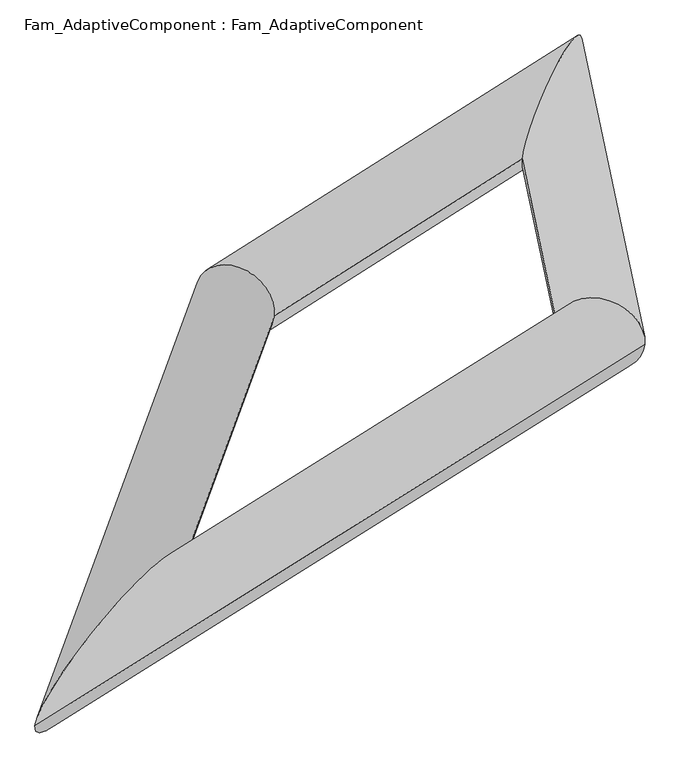
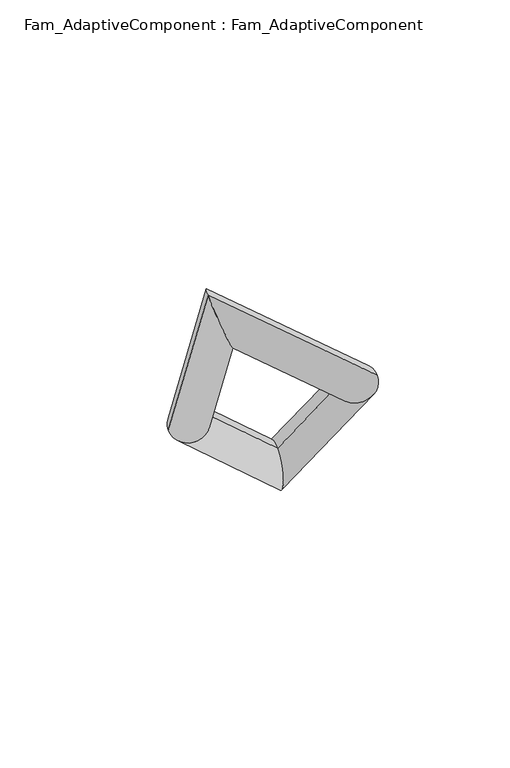
"""IFC4 building model written with IfcOpenShell, lengths in millimetres: proxy geometry, Fam_AdaptiveComponent : Fam_AdaptiveComponent."""

from ifc_helpers import new_model, si_unit, frame, origin, place, context, project, spatial, ellipse_curve, source, transform, mapped, element, save
from ifc_brep_helpers import cylinder_surface, advanced_brep


def fam_adaptivecomponent_fam_adaptivecomponent_cf6aee74(model_context):
    return source(origin(), model_context, "Body", "AdvancedBrep", [
        advanced_brep(
        [(4475.999331, 1861.8658467, -16792.1550666), (3077.0233369, 8482.3914405, -26020.1836237), (5467.6276173, 13102.4870202, -32934.2739452), (8018.1342606, 1032.4482346, -16110.4340521), (-6896.2487487, 2172.9196503, -15463.0140025), (-10041.8321805, 3290.6120172, -16516.7936626), (-10452.4436557, -7477.6518919, -1139.2130585), (-16534.2015959, -14327.9598441, 9633.4623253)],
        [
            (0, 1),
            (1, 2, ellipse_curve(frame((4272.3254771, 10792.4392303, -29477.2287844), z_axis=(0.9570179583452368, -0.22916247099373624, 0.17776723346207376), x_axis=(-0.27599610140512587, -0.5312433964626994, 0.8010034991958193)), 4326.3578156, 1700.0)),
            (2, 3),
            (3, 0, ellipse_curve(frame((6247.0667958, 1447.1570406, -16451.2945594), z_axis=(0.27834003989802747, 0.5306803364613102, -0.8005655517712932), x_axis=(0.9563388744454964, -0.23046336995386144, 0.17972921947705384)), 1850.6452556, 1700.0)),
            (2, 1, ellipse_curve(frame((4272.3254771, 10792.4392303, -29477.2287844), z_axis=(0.9570179583452368, -0.22916247099373624, 0.17776723346207376), x_axis=(-0.27599610140512587, -0.5312433964626994, 0.8010034991958193)), 4326.3578156, 1700.0)),
            (0, 3, ellipse_curve(frame((6247.0667958, 1447.1570406, -16451.2945594), z_axis=(0.27834003989802747, 0.5306803364613102, -0.8005655517712932), x_axis=(0.9563388744454964, -0.23046336995386144, 0.17972921947705384)), 1850.6452556, 1700.0)),
            (1, 4),
            (4, 5, ellipse_curve(frame((-8469.0404646, 2731.7658338, -15989.9038326), z_axis=(0.4280636238956785, 0.4868668836941716, -0.7613948853645033), x_axis=(0.8993435130601728, -0.31256298878643, 0.3057541881274575)), 1750.3166187, 1700.0)),
            (5, 2),
            (5, 4, ellipse_curve(frame((-8469.0404646, 2731.7658338, -15989.9038326), z_axis=(0.4280636238956785, 0.4868668836941716, -0.7613948853645033), x_axis=(0.8993435130601728, -0.31256298878643, 0.3057541881274575)), 1750.3166187, 1700.0)),
            (4, 6),
            (6, 7, ellipse_curve(frame((-13493.3226258, -10902.805868, 4247.1246334), z_axis=(-0.8982920252561902, 0.3137549115890715, -0.3076187458768823), x_axis=(0.43026579918376734, 0.48609961926637424, -0.7606434790372163)), 7070.6901554, 1700.0)),
            (7, 5),
            (7, 6, ellipse_curve(frame((-13493.3226258, -10902.805868, 4247.1246334), z_axis=(-0.8982920252561902, 0.3137549115890715, -0.3076187458768823), x_axis=(0.43026579918376734, 0.48609961926637424, -0.7606434790372163)), 7070.6901554, 1700.0)),
            (6, 0),
            (3, 7),
        ],
        [
            cylinder_surface(frame((6247.0667958, 1447.1570406, -16451.2945594), z_axis=(0.1222547651073129, -0.5785594640476796, 0.8064258918024754), x_axis=(0.8331796388730955, 0.5013465746799647, 0.23337373764835828)), 1700.0),
            cylinder_surface(frame((4272.3254771, 10792.4392303, -29477.2287844), z_axis=(0.6298469326773338, 0.39846515965142004, -0.6667220994844273), x_axis=(-0.5525139586135777, 0.833157452491823, -0.024020509871553453)), 1700.0),
            cylinder_surface(frame((-8469.0404646, 2731.7658338, -15989.9038326), z_axis=(0.20166909460392543, 0.5472765346786865, -0.8122918015539253), x_axis=(-0.7129648228847512, 0.6506653931039864, 0.26137273680655826)), 1700.0),
            cylinder_surface(frame((-13493.3226258, -10902.805868, 4247.1246334), z_axis=(-0.6336202646810969, -0.39640488340280305, 0.6643707764493157), x_axis=(0.6599791823502691, 0.1711243164074559, 0.731535335577408)), 1700.0),
        ],
        [
            (0, [[1, 2, 3, 4]]),
            (0, [[-3, 5, -1, 6]]),
            (1, [[7, 8, 9, -2]]),
            (1, [[-9, 10, -7, -5]]),
            (2, [[11, 12, 13, -8]]),
            (2, [[-13, 14, -11, -10]]),
            (3, [[15, -4, 16, -12]]),
            (3, [[-16, -6, -15, -14]]),
        ],
    ),
    ])


if __name__ == "__main__":
    model = new_model("IFC4")
    model_context = context("Model", 3, world=origin())
    ifc_project = project(units=[si_unit("LENGTHUNIT", "METRE", prefix="MILLI")], contexts=[model_context])
    site = spatial("IfcSite", under=ifc_project)
    building = spatial("IfcBuilding", under=site)
    placement = place(None, origin())
    fam_adaptivecomponent_fam_adaptivecomponent_shape = fam_adaptivecomponent_fam_adaptivecomponent_cf6aee74(model_context)
    element("IfcBuildingElementProxy", 1, Name="Fam_AdaptiveComponent : Fam_AdaptiveComponent", ObjectType="Fam_AdaptiveComponent : Fam_AdaptiveComponent", at=placement, inside=building, context=model_context, shape_type="MappedRepresentation", body=[
        mapped(fam_adaptivecomponent_fam_adaptivecomponent_shape, transform((0.0, 0.0, 0.0), x_axis=(1.0, 0.0, 0.0), y_axis=(0.0, 1.0, 0.0), z_axis=(0.0, 0.0, 1.0))),
    ])
    save(model, "model.ifc")

# Revit data of these elements
# Project information
#   Project Issue Date = "Issue Date"
#   Project Status = "Project Status"
#   Client Name = "Owner"
#   Project Address = "Enter address here"
#   Project Name = "Project Name"
#   Project Number = "0001"
# Type "Fam_AdaptiveComponent : Fam_AdaptiveComponent"
#   Default Elevation = 0
